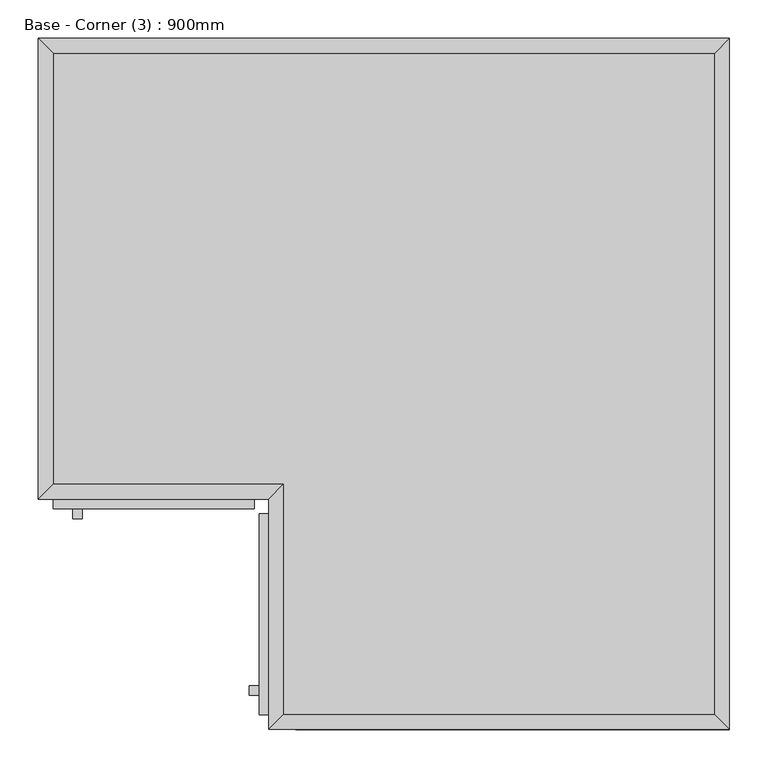
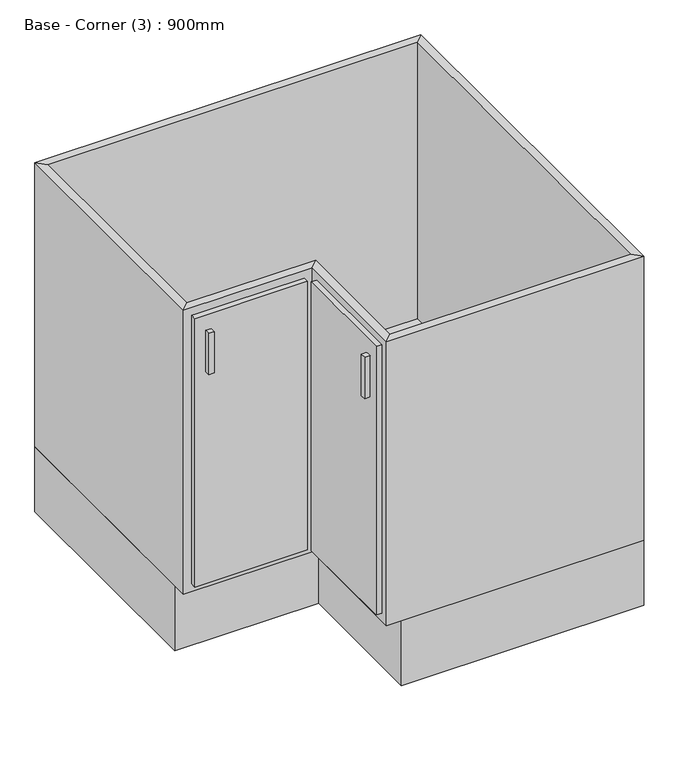
"""IFC4 building model written with IfcOpenShell, lengths in millimetres: furniture geometry, Base - Corner (3) : 900mm."""

import ifcopenshell
import ifcopenshell.guid

model = None  # the IFC model being written
_history = None  # IfcOwnerHistory: only IFC2X3 demands one
_inside = {}  # id of a spatial element -> (the spatial element, [elements in it])
_under = {}  # id of a project, library or spatial element -> (it, [spatial elements below it])
_declared = {}  # id of a project -> (the project, [libraries it declares])
_typed = {}  # id of a type object -> (the type object, [elements of that type])
_made_of = {}  # id of a material, layer set ... -> (it, [elements and type objects made of it])


def new_model(schema):
    """Start an empty IFC model of exactly this schema.

    Asked for "IFC4X3", IfcOpenShell would pick the latest addendum, in which some entities
    have other attributes; the version numbers below select the first issue.
    IFC2X3 requires an IfcOwnerHistory on every rooted entity: one is made here for all.
    """
    global model, _history
    if schema == "IFC4X3":
        model = ifcopenshell.file(schema_version=(4, 3, 0, 0))
    else:
        model = ifcopenshell.file(schema=schema)
    _inside.clear()
    _under.clear()
    _declared.clear()
    _typed.clear()
    _made_of.clear()
    _history = None
    if model.schema == "IFC2X3":
        org = make("IfcOrganization", Name="unknown")
        user = make(
            "IfcPersonAndOrganization",
            ThePerson=make("IfcPerson", FamilyName="unknown"),
            TheOrganization=org,
        )
        app = make(
            "IfcApplication",
            ApplicationDeveloper=org,
            Version="unknown",
            ApplicationFullName="unknown",
            ApplicationIdentifier="unknown",
        )
        _history = make(
            "IfcOwnerHistory",
            OwningUser=user,
            OwningApplication=app,
            ChangeAction="ADDED",
            CreationDate=0,
        )
    return model


def make(cls, **values):
    """One entity of the class cls with the attributes given. An attribute that is None is left unset."""
    return model.create_entity(
        cls, **{name: value for name, value in values.items() if value is not None}
    )


def rooted(cls, **values):
    """An entity with a GlobalId (a new one), such as an element, a storey or a relation."""
    return make(cls, GlobalId=ifcopenshell.guid.new(), OwnerHistory=_history, **values)


def si_unit(unit_type, name, prefix=None):
    """IfcSIUnit, for example si_unit("LENGTHUNIT", "METRE", prefix="MILLI")."""
    return make("IfcSIUnit", UnitType=unit_type, Prefix=prefix, Name=name)


def assignment(units):
    """IfcUnitAssignment: the units of a project."""
    return None if units is None else make("IfcUnitAssignment", Units=units)


def point(xyz):
    """IfcCartesianPoint."""
    return None if xyz is None else make("IfcCartesianPoint", Coordinates=xyz)


def direction(xyz):
    """IfcDirection."""
    return None if xyz is None else make("IfcDirection", DirectionRatios=xyz)


def frame(location, z_axis=None, x_axis=None):
    """IfcAxis2Placement3D, a coordinate frame: its origin and axes. An axis left out is left unset."""
    return make(
        "IfcAxis2Placement3D",
        Location=point(location),
        Axis=direction(z_axis),
        RefDirection=direction(x_axis),
    )


def origin():
    """The frame at (0, 0, 0) with its axes left unset."""
    return frame((0.0, 0.0, 0.0))


def origin_with_axes():
    """The frame at (0, 0, 0) with the z axis (0, 0, 1) and the x axis (1, 0, 0) written out."""
    return frame((0.0, 0.0, 0.0), z_axis=(0.0, 0.0, 1.0), x_axis=(1.0, 0.0, 0.0))


def place(relative_to, where):
    """IfcLocalPlacement: puts the frame where relative to a parent placement (None: the world)."""
    return make(
        "IfcLocalPlacement", PlacementRelTo=relative_to, RelativePlacement=where
    )


def context(
    kind, dimensions, precision=None, world=None, true_north=None, identifier=None
):
    """IfcGeometricRepresentationContext, for example the 3D "Model" context."""
    return make(
        "IfcGeometricRepresentationContext",
        ContextIdentifier=identifier,
        ContextType=kind,
        CoordinateSpaceDimension=dimensions,
        Precision=precision,
        WorldCoordinateSystem=world,
        TrueNorth=true_north,
    )


def project(units=None, contexts=None):
    """IfcProject with its units and contexts."""
    return rooted(
        "IfcProject",
        Name="project",
        RepresentationContexts=contexts,
        UnitsInContext=assignment(units),
    )


def spatial(cls, under=None, at=None, **own):
    """A site, building, storey or space (cls), placed at a placement, below another one or the project."""
    s = rooted(cls, ObjectPlacement=at, **own)
    if under is not None:
        _under.setdefault(under.id(), (under, []))[1].append(s)
    return s


def polyline(points):
    """IfcPolyline through the points."""
    return make("IfcPolyline", Points=[point(p) for p in points])


def outline(outer, holes=None, kind="AREA"):
    """IfcArbitraryClosedProfileDef: a profile drawn as a closed curve; with holes, ...WithVoids."""
    if holes is None:
        return make("IfcArbitraryClosedProfileDef", ProfileType=kind, OuterCurve=outer)
    return make(
        "IfcArbitraryProfileDefWithVoids",
        ProfileType=kind,
        OuterCurve=outer,
        InnerCurves=holes,
    )


def extrude(swept, where, along, depth):
    """IfcExtrudedAreaSolid: the profile swept, set in the frame where, extruded along a direction by depth."""
    return make(
        "IfcExtrudedAreaSolid",
        SweptArea=swept,
        Position=where,
        ExtrudedDirection=direction(along),
        Depth=depth,
    )


def faces_of(points, faces, orient=None, outer=None):
    """IfcFace entities. A face is a list of loops; a loop is a list of indices into points, from 0.

    orient and outer hold one flag for each loop. By default every Orientation is true, the
    first loop of a face is its IfcFaceOuterBound and the others are IfcFaceBound.
    """
    made = []
    for i, loops in enumerate(faces):
        bounds = []
        for j, loop in enumerate(loops):
            is_outer = j == 0 if outer is None else outer[i][j]
            bounds.append(
                make(
                    "IfcFaceOuterBound" if is_outer else "IfcFaceBound",
                    Bound=make("IfcPolyLoop", Polygon=[points[k] for k in loop]),
                    Orientation=True if orient is None else orient[i][j],
                )
            )
        made.append(make("IfcFace", Bounds=bounds))
    return made


def faceted_brep(points, faces, orient=None, outer=None, voids=None):
    """IfcFacetedBrep: a solid bounded by flat faces; with voids (closed shells), ...WithVoids."""
    shared = [point(p) for p in points]
    hull = make("IfcClosedShell", CfsFaces=faces_of(shared, faces, orient, outer))
    if voids is None:
        return make("IfcFacetedBrep", Outer=hull)
    return make(
        "IfcFacetedBrepWithVoids",
        Outer=hull,
        Voids=[
            make(cls, CfsFaces=faces_of(shared, fs, o, b)) for cls, fs, o, b in voids
        ],
    )


def shape(context_of_items, identifier, shape_type, items):
    """IfcShapeRepresentation: the items that make up one representation, for example the "Body"."""
    return make(
        "IfcShapeRepresentation",
        ContextOfItems=context_of_items,
        RepresentationIdentifier=identifier,
        RepresentationType=shape_type,
        Items=items,
    )


def source(mapping_origin, context_of_items, identifier, shape_type, items):
    """IfcRepresentationMap: a shape defined once, which mapped items show again and again."""
    return make(
        "IfcRepresentationMap",
        MappingOrigin=mapping_origin,
        MappedRepresentation=shape(context_of_items, identifier, shape_type, items),
    )


def transform(
    local_origin,
    x_axis=None,
    y_axis=None,
    z_axis=None,
    scale=None,
    scale2=None,
    scale3=None,
    uniform=True,
):
    """IfcCartesianTransformationOperator3D, or its non-uniform kind. x_axis, y_axis, z_axis: its Axis1, 2, 3."""
    if uniform:
        return make(
            "IfcCartesianTransformationOperator3D",
            Axis1=direction(x_axis),
            Axis2=direction(y_axis),
            LocalOrigin=point(local_origin),
            Scale=scale,
            Axis3=direction(z_axis),
        )
    return make(
        "IfcCartesianTransformationOperator3DnonUniform",
        Axis1=direction(x_axis),
        Axis2=direction(y_axis),
        LocalOrigin=point(local_origin),
        Scale=scale,
        Axis3=direction(z_axis),
        Scale2=scale2,
        Scale3=scale3,
    )


def mapped(mapping_source, mapping_target):
    """IfcMappedItem: shows the shape of a source again, moved by a transform."""
    return make(
        "IfcMappedItem", MappingSource=mapping_source, MappingTarget=mapping_target
    )


def made_of(thing, what):
    """Note that an element or type object is made of a material, layer set ...; save() writes the relation."""
    if what is not None:
        _made_of.setdefault(what.id(), (what, []))[1].append(thing)
    return thing


def element(
    cls,
    number,
    at=None,
    inside=None,
    cuts=None,
    type_object=None,
    material=None,
    context=None,
    identifier="Body",
    shape_type=None,
    held_by="IfcProductDefinitionShape",
    body=None,
    shapes=None,
    **own,
):
    """One element of the class cls, such as IfcWall. Its Tag is "e" and its number.

    at: its placement. inside: the storey or other place that contains it. cuts: it is an
    opening in that element (IfcRelVoidsElement). A single representation is given by context,
    identifier, shape_type and body (its items); several are given by shapes. held_by: the class
    of the entity that holds the representations. save() writes the other relations.
    """
    e = rooted(cls, Tag="e%d" % number, ObjectPlacement=at, **own)
    if body is not None:
        shapes = [shape(context, identifier, shape_type, body)]
    if shapes is not None:
        e.Representation = make(held_by, Representations=shapes)
    if inside is not None:
        _inside.setdefault(inside.id(), (inside, []))[1].append(e)
    if cuts is not None:
        rooted(
            "IfcRelVoidsElement", RelatingBuildingElement=cuts, RelatedOpeningElement=e
        )
    if type_object is not None:
        _typed.setdefault(type_object.id(), (type_object, []))[1].append(e)
    return made_of(e, material)


def aggregate(whole, parts):
    """IfcRelAggregates: a whole, such as a stair, and the parts it consists of."""
    return rooted("IfcRelAggregates", RelatingObject=whole, RelatedObjects=parts)


def save(model, path):
    """Write the relations noted so far, then the file.

    IfcRelAggregates (storeys below a building ...), IfcRelContainedInSpatialStructure (elements
    in a storey), IfcRelDefinesByType, IfcRelAssociatesMaterial and IfcRelDeclares: one each for
    every whole, place, type object, material and project.
    """
    for whole, parts in _under.values():
        aggregate(whole, parts)
    for where, things in _inside.values():
        rooted(
            "IfcRelContainedInSpatialStructure",
            RelatedElements=things,
            RelatingStructure=where,
        )
    for kind, things in _typed.values():
        rooted("IfcRelDefinesByType", RelatedObjects=things, RelatingType=kind)
    for what, things in _made_of.values():
        rooted("IfcRelAssociatesMaterial", RelatedObjects=things, RelatingMaterial=what)
    for by, libraries in _declared.values():
        rooted("IfcRelDeclares", RelatingContext=by, RelatedDefinitions=libraries)
    model.write(path)


def base_corner_3_900mm_cbc719dc(model_context):
    return source(origin(), model_context, "Body", "SolidModel", [
        extrude(outline(polyline([(-100.3622951, -842.85), (-100.3622951, -855.55), (-113.0622951, -855.55), (-113.0622951, -842.85), (-100.3622951, -842.85)])), frame((0.0, 0.0, 701.25), z_axis=(0.0, 0.0, 1.0), x_axis=(1.0, 0.0, 0.0)), (0.0, 0.0, 1.0), 101.6),
        extrude(outline(polyline([(-87.6622951, -619.05), (-87.6622951, -880.95), (-100.3622951, -880.95), (-100.3622951, -619.05), (-87.6622951, -619.05)])), frame((0.0, 0.0, 179.05), z_axis=(0.0, 0.0, 1.0), x_axis=(1.0, 0.0, 0.0)), (0.0, 0.0, 1.0), 661.9),
        extrude(outline(polyline([(-330.5122951, -625.4), (-343.2122951, -625.4), (-343.2122951, -612.7), (-330.5122951, -612.7), (-330.5122951, -625.4)])), frame((0.0, 0.0, 701.25), z_axis=(0.0, 0.0, 1.0), x_axis=(1.0, 0.0, 0.0)), (0.0, 0.0, 1.0), 101.6),
        extrude(outline(polyline([(-106.7122951, -612.7), (-368.6122951, -612.7), (-368.6122951, -600.0), (-106.7122951, -600.0), (-106.7122951, -612.7)])), frame((0.0, 0.0, 179.05), z_axis=(0.0, 0.0, 1.0), x_axis=(1.0, 0.0, 0.0)), (0.0, 0.0, 1.0), 661.9),
        faceted_brep([(493.2877049, -880.95, 860.0), (493.2877049, -880.95, 160.0), (-68.6122951, -880.95, 160.0), (-68.6122951, -880.95, 860.0), (512.3377049, -900.0, 860.0), (-87.6622951, -900.0, 860.0), (512.3377049, -900.0, 160.0), (-87.6622951, -900.0, 160.0), (-68.6122951, -580.95, 160.0), (-68.6122951, -580.95, 860.0), (-87.6622951, -600.0, 860.0), (-87.6622951, -600.0, 160.0), (-368.6122951, -580.95, 160.0), (-368.6122951, -580.95, 860.0), (-387.6622951, -600.0, 860.0), (-387.6622951, -600.0, 160.0), (-368.6122951, -19.05, 160.0), (-368.6122951, -19.05, 860.0), (-387.6622951, 0.0, 860.0), (-387.6622951, 0.0, 160.0), (493.2877049, -19.05, 160.0), (493.2877049, -19.05, 860.0), (512.3377049, 0.0, 860.0), (512.3377049, 0.0, 160.0)], [[[0, 1, 2, 3]], [[4, 0, 3, 5]], [[6, 4, 5, 7]], [[1, 6, 7, 2]], [[3, 2, 8, 9]], [[5, 3, 9, 10]], [[7, 5, 10, 11]], [[2, 7, 11, 8]], [[9, 8, 12, 13]], [[10, 9, 13, 14]], [[11, 10, 14, 15]], [[8, 11, 15, 12]], [[13, 12, 16, 17]], [[14, 13, 17, 18]], [[15, 14, 18, 19]], [[12, 15, 19, 16]], [[17, 16, 20, 21]], [[18, 17, 21, 22]], [[19, 18, 22, 23]], [[16, 19, 23, 20]], [[21, 20, 1, 0]], [[22, 21, 0, 4]], [[23, 22, 4, 6]], [[20, 23, 6, 1]]]),
        extrude(outline(polyline([(493.2877049, -19.05), (493.2877049, -880.95), (-68.6122951, -880.95), (-68.6122951, -580.95), (-368.6122951, -580.95), (-368.6122951, -19.05), (493.2877049, -19.05)])), frame((0.0, 0.0, 160.0), z_axis=(0.0, 0.0, 1.0), x_axis=(1.0, 0.0, 0.0)), (0.0, 0.0, 1.0), 19.05),
        extrude(outline(polyline([(512.3377049, 0.0), (512.3377049, -900.0), (-52.6622951, -900.0), (-52.6622951, -565.0), (-387.6622951, -565.0), (-387.6622951, 0.0), (512.3377049, 0.0)])), origin_with_axes(), (0.0, 0.0, 1.0), 160.0),
    ])


if __name__ == "__main__":
    model = new_model("IFC4")
    model_context = context("Model", 3, world=origin())
    ifc_project = project(units=[si_unit("LENGTHUNIT", "METRE", prefix="MILLI")], contexts=[model_context])
    site = spatial("IfcSite", under=ifc_project)
    building = spatial("IfcBuilding", under=site)
    placement = place(None, origin())
    base_corner_3_900mm_shape = base_corner_3_900mm_cbc719dc(model_context)
    element("IfcFurniture", 1, ObjectType="Base - Corner (3) : 900mm", at=placement, inside=building, context=model_context, shape_type="MappedRepresentation", body=[
        mapped(base_corner_3_900mm_shape, transform((0.0, 0.0, 0.0), x_axis=(1.0, 0.0, 0.0), y_axis=(0.0, 1.0, 0.0), z_axis=(0.0, 0.0, 1.0))),
    ])
    save(model, "model.ifc")

# Revit data of these elements
# Type "Base - Corner (3) : 900mm"
#   Keynote = "N10"
#   Depth = 600 mm
#   Height = 860 mm
#   Toe Depth = 35 mm
#   Toe Height = 160 mm
#   Width = 900 mm
#   Cabinet Material = Cabinets
#   Door/Drawer Material = Cabinets
#   Handle Material = Cabinets - Handles
#   Default Elevation = 0
#   Assembly Code = ""
# Element 1 (IfcFurniture, "Base - Corner (3) : 900mm")
#   Materials on its faces: "Cabinets", "Cabinets - Handles"
# Materials
#   "Cabinets": class "Miscellaneous", colour RGB 249 249 249, transparency 0
#   "Cabinets - Handles": class "Metal", colour RGB 57 57 57, transparency 0
